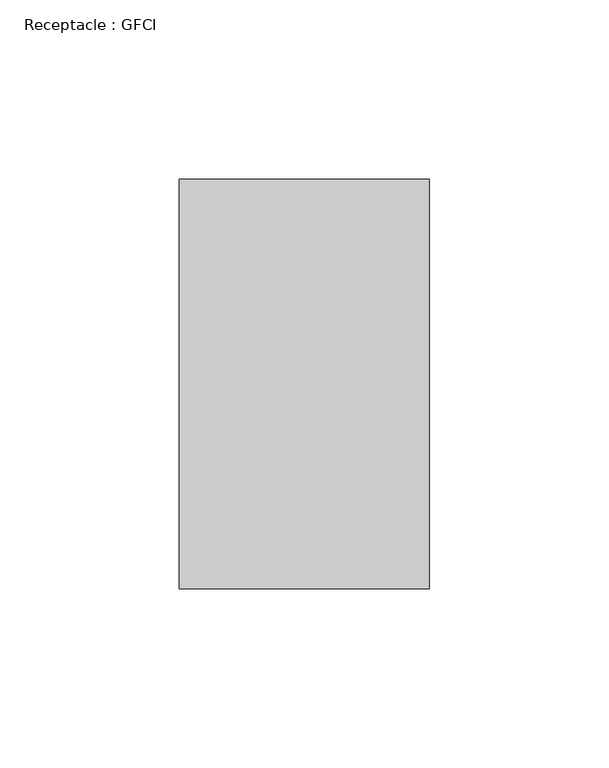
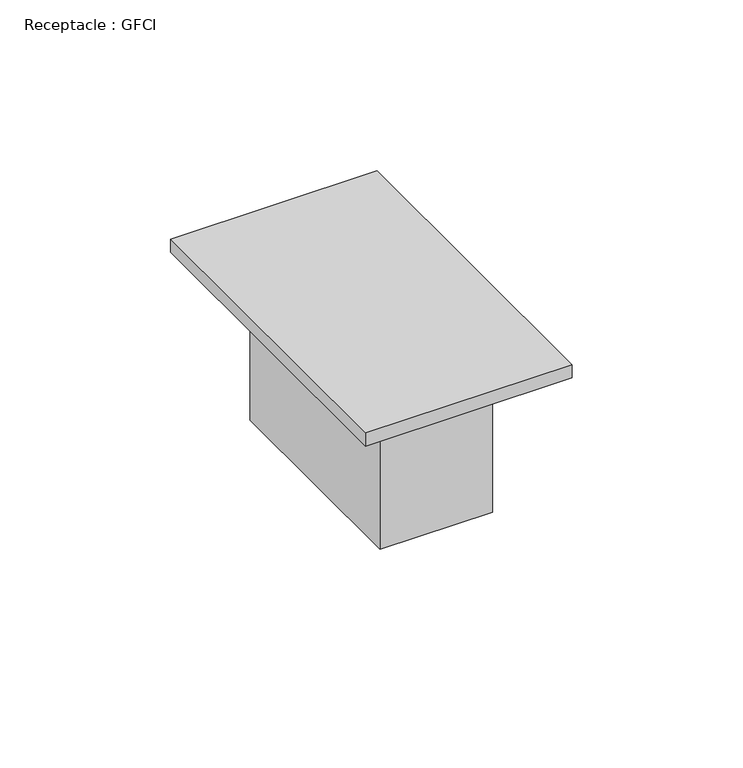
"""IFC4 building model written with IfcOpenShell, lengths in millimetres: proxy geometry, Receptacle : GFCI."""

import ifcopenshell
import ifcopenshell.guid

model = None  # the IFC model being written
_history = None  # IfcOwnerHistory: only IFC2X3 demands one
_inside = {}  # id of a spatial element -> (the spatial element, [elements in it])
_under = {}  # id of a project, library or spatial element -> (it, [spatial elements below it])
_declared = {}  # id of a project -> (the project, [libraries it declares])
_typed = {}  # id of a type object -> (the type object, [elements of that type])
_made_of = {}  # id of a material, layer set ... -> (it, [elements and type objects made of it])


def new_model(schema):
    """Start an empty IFC model of exactly this schema.

    Asked for "IFC4X3", IfcOpenShell would pick the latest addendum, in which some entities
    have other attributes; the version numbers below select the first issue.
    IFC2X3 requires an IfcOwnerHistory on every rooted entity: one is made here for all.
    """
    global model, _history
    if schema == "IFC4X3":
        model = ifcopenshell.file(schema_version=(4, 3, 0, 0))
    else:
        model = ifcopenshell.file(schema=schema)
    _inside.clear()
    _under.clear()
    _declared.clear()
    _typed.clear()
    _made_of.clear()
    _history = None
    if model.schema == "IFC2X3":
        org = make("IfcOrganization", Name="unknown")
        user = make(
            "IfcPersonAndOrganization",
            ThePerson=make("IfcPerson", FamilyName="unknown"),
            TheOrganization=org,
        )
        app = make(
            "IfcApplication",
            ApplicationDeveloper=org,
            Version="unknown",
            ApplicationFullName="unknown",
            ApplicationIdentifier="unknown",
        )
        _history = make(
            "IfcOwnerHistory",
            OwningUser=user,
            OwningApplication=app,
            ChangeAction="ADDED",
            CreationDate=0,
        )
    return model


def make(cls, **values):
    """One entity of the class cls with the attributes given. An attribute that is None is left unset."""
    return model.create_entity(
        cls, **{name: value for name, value in values.items() if value is not None}
    )


def rooted(cls, **values):
    """An entity with a GlobalId (a new one), such as an element, a storey or a relation."""
    return make(cls, GlobalId=ifcopenshell.guid.new(), OwnerHistory=_history, **values)


def si_unit(unit_type, name, prefix=None):
    """IfcSIUnit, for example si_unit("LENGTHUNIT", "METRE", prefix="MILLI")."""
    return make("IfcSIUnit", UnitType=unit_type, Prefix=prefix, Name=name)


def assignment(units):
    """IfcUnitAssignment: the units of a project."""
    return None if units is None else make("IfcUnitAssignment", Units=units)


def point(xyz):
    """IfcCartesianPoint."""
    return None if xyz is None else make("IfcCartesianPoint", Coordinates=xyz)


def direction(xyz):
    """IfcDirection."""
    return None if xyz is None else make("IfcDirection", DirectionRatios=xyz)


def frame(location, z_axis=None, x_axis=None):
    """IfcAxis2Placement3D, a coordinate frame: its origin and axes. An axis left out is left unset."""
    return make(
        "IfcAxis2Placement3D",
        Location=point(location),
        Axis=direction(z_axis),
        RefDirection=direction(x_axis),
    )


def origin():
    """The frame at (0, 0, 0) with its axes left unset."""
    return frame((0.0, 0.0, 0.0))


def origin_with_axes():
    """The frame at (0, 0, 0) with the z axis (0, 0, 1) and the x axis (1, 0, 0) written out."""
    return frame((0.0, 0.0, 0.0), z_axis=(0.0, 0.0, 1.0), x_axis=(1.0, 0.0, 0.0))


def place(relative_to, where):
    """IfcLocalPlacement: puts the frame where relative to a parent placement (None: the world)."""
    return make(
        "IfcLocalPlacement", PlacementRelTo=relative_to, RelativePlacement=where
    )


def context(
    kind, dimensions, precision=None, world=None, true_north=None, identifier=None
):
    """IfcGeometricRepresentationContext, for example the 3D "Model" context."""
    return make(
        "IfcGeometricRepresentationContext",
        ContextIdentifier=identifier,
        ContextType=kind,
        CoordinateSpaceDimension=dimensions,
        Precision=precision,
        WorldCoordinateSystem=world,
        TrueNorth=true_north,
    )


def project(units=None, contexts=None):
    """IfcProject with its units and contexts."""
    return rooted(
        "IfcProject",
        Name="project",
        RepresentationContexts=contexts,
        UnitsInContext=assignment(units),
    )


def spatial(cls, under=None, at=None, **own):
    """A site, building, storey or space (cls), placed at a placement, below another one or the project."""
    s = rooted(cls, ObjectPlacement=at, **own)
    if under is not None:
        _under.setdefault(under.id(), (under, []))[1].append(s)
    return s


def polyline(points):
    """IfcPolyline through the points."""
    return make("IfcPolyline", Points=[point(p) for p in points])


def outline(outer, holes=None, kind="AREA"):
    """IfcArbitraryClosedProfileDef: a profile drawn as a closed curve; with holes, ...WithVoids."""
    if holes is None:
        return make("IfcArbitraryClosedProfileDef", ProfileType=kind, OuterCurve=outer)
    return make(
        "IfcArbitraryProfileDefWithVoids",
        ProfileType=kind,
        OuterCurve=outer,
        InnerCurves=holes,
    )


def extrude(swept, where, along, depth):
    """IfcExtrudedAreaSolid: the profile swept, set in the frame where, extruded along a direction by depth."""
    return make(
        "IfcExtrudedAreaSolid",
        SweptArea=swept,
        Position=where,
        ExtrudedDirection=direction(along),
        Depth=depth,
    )


def shape(context_of_items, identifier, shape_type, items):
    """IfcShapeRepresentation: the items that make up one representation, for example the "Body"."""
    return make(
        "IfcShapeRepresentation",
        ContextOfItems=context_of_items,
        RepresentationIdentifier=identifier,
        RepresentationType=shape_type,
        Items=items,
    )


def source(mapping_origin, context_of_items, identifier, shape_type, items):
    """IfcRepresentationMap: a shape defined once, which mapped items show again and again."""
    return make(
        "IfcRepresentationMap",
        MappingOrigin=mapping_origin,
        MappedRepresentation=shape(context_of_items, identifier, shape_type, items),
    )


def transform(
    local_origin,
    x_axis=None,
    y_axis=None,
    z_axis=None,
    scale=None,
    scale2=None,
    scale3=None,
    uniform=True,
):
    """IfcCartesianTransformationOperator3D, or its non-uniform kind. x_axis, y_axis, z_axis: its Axis1, 2, 3."""
    if uniform:
        return make(
            "IfcCartesianTransformationOperator3D",
            Axis1=direction(x_axis),
            Axis2=direction(y_axis),
            LocalOrigin=point(local_origin),
            Scale=scale,
            Axis3=direction(z_axis),
        )
    return make(
        "IfcCartesianTransformationOperator3DnonUniform",
        Axis1=direction(x_axis),
        Axis2=direction(y_axis),
        LocalOrigin=point(local_origin),
        Scale=scale,
        Axis3=direction(z_axis),
        Scale2=scale2,
        Scale3=scale3,
    )


def mapped(mapping_source, mapping_target):
    """IfcMappedItem: shows the shape of a source again, moved by a transform."""
    return make(
        "IfcMappedItem", MappingSource=mapping_source, MappingTarget=mapping_target
    )


def made_of(thing, what):
    """Note that an element or type object is made of a material, layer set ...; save() writes the relation."""
    if what is not None:
        _made_of.setdefault(what.id(), (what, []))[1].append(thing)
    return thing


def element(
    cls,
    number,
    at=None,
    inside=None,
    cuts=None,
    type_object=None,
    material=None,
    context=None,
    identifier="Body",
    shape_type=None,
    held_by="IfcProductDefinitionShape",
    body=None,
    shapes=None,
    **own,
):
    """One element of the class cls, such as IfcWall. Its Tag is "e" and its number.

    at: its placement. inside: the storey or other place that contains it. cuts: it is an
    opening in that element (IfcRelVoidsElement). A single representation is given by context,
    identifier, shape_type and body (its items); several are given by shapes. held_by: the class
    of the entity that holds the representations. save() writes the other relations.
    """
    e = rooted(cls, Tag="e%d" % number, ObjectPlacement=at, **own)
    if body is not None:
        shapes = [shape(context, identifier, shape_type, body)]
    if shapes is not None:
        e.Representation = make(held_by, Representations=shapes)
    if inside is not None:
        _inside.setdefault(inside.id(), (inside, []))[1].append(e)
    if cuts is not None:
        rooted(
            "IfcRelVoidsElement", RelatingBuildingElement=cuts, RelatedOpeningElement=e
        )
    if type_object is not None:
        _typed.setdefault(type_object.id(), (type_object, []))[1].append(e)
    return made_of(e, material)


def aggregate(whole, parts):
    """IfcRelAggregates: a whole, such as a stair, and the parts it consists of."""
    return rooted("IfcRelAggregates", RelatingObject=whole, RelatedObjects=parts)


def save(model, path):
    """Write the relations noted so far, then the file.

    IfcRelAggregates (storeys below a building ...), IfcRelContainedInSpatialStructure (elements
    in a storey), IfcRelDefinesByType, IfcRelAssociatesMaterial and IfcRelDeclares: one each for
    every whole, place, type object, material and project.
    """
    for whole, parts in _under.values():
        aggregate(whole, parts)
    for where, things in _inside.values():
        rooted(
            "IfcRelContainedInSpatialStructure",
            RelatedElements=things,
            RelatingStructure=where,
        )
    for kind, things in _typed.values():
        rooted("IfcRelDefinesByType", RelatedObjects=things, RelatingType=kind)
    for what, things in _made_of.values():
        rooted("IfcRelAssociatesMaterial", RelatedObjects=things, RelatingMaterial=what)
    for by, libraries in _declared.values():
        rooted("IfcRelDeclares", RelatingContext=by, RelatedDefinitions=libraries)
    model.write(path)


def receptacle_gfci_367a9a66(model_context):
    return source(origin(), model_context, "Body", "SweptSolid", [
        extrude(outline(polyline([(34.925, 57.15), (34.925, -57.15), (-34.925, -57.15), (-34.925, 57.15), (34.925, 57.15)])), origin_with_axes(), (0.0, 0.0, 1.0), 4.7625),
        extrude(outline(polyline([(19.05, 38.1), (19.05, -38.1), (-19.05, -38.1), (-19.05, 38.1), (19.05, 38.1)])), frame((0.0, 0.0, -53.975), z_axis=(0.0, 0.0, 1.0), x_axis=(1.0, 0.0, 0.0)), (0.0, 0.0, 1.0), 53.975),
    ])


if __name__ == "__main__":
    model = new_model("IFC4")
    model_context = context("Model", 3, world=origin())
    ifc_project = project(units=[si_unit("LENGTHUNIT", "METRE", prefix="MILLI")], contexts=[model_context])
    site = spatial("IfcSite", under=ifc_project)
    building = spatial("IfcBuilding", under=site)
    placement = place(None, origin())
    receptacle_gfci_shape = receptacle_gfci_367a9a66(model_context)
    element("IfcBuildingElementProxy", 1, Name="Receptacle : GFCI", ObjectType="Receptacle : GFCI", at=placement, inside=building, context=model_context, shape_type="MappedRepresentation", body=[
        mapped(receptacle_gfci_shape, transform((0.0, 0.0, 0.0), x_axis=(1.0, 0.0, 0.0), y_axis=(0.0, 1.0, 0.0), z_axis=(0.0, 0.0, 1.0))),
    ])
    save(model, "model.ifc")

# Revit data of these elements
# Type "Receptacle : GFCI"
#   Label = "GFCI"
#   Switch Voltage = 120 V
#   Load = 180 VA
#   Default Elevation = 4' - 0"
#   FacePlate = none
#   Assembly Code = ""
